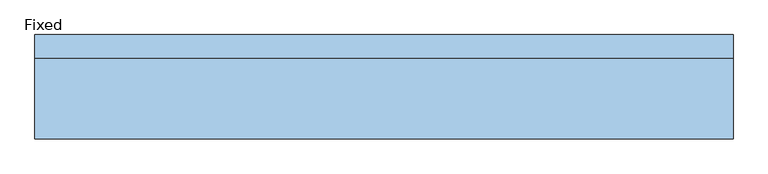
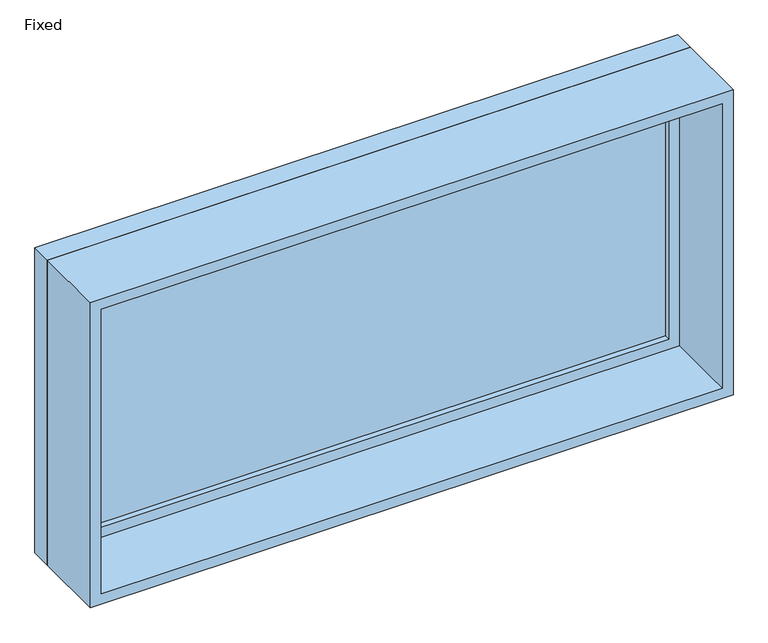
"""IFC4 building model written with IfcOpenShell, lengths in millimetres: window geometry, Fixed."""

import ifcopenshell
import ifcopenshell.guid

model = None  # the IFC model being written
_history = None  # IfcOwnerHistory: only IFC2X3 demands one
_inside = {}  # id of a spatial element -> (the spatial element, [elements in it])
_under = {}  # id of a project, library or spatial element -> (it, [spatial elements below it])
_declared = {}  # id of a project -> (the project, [libraries it declares])
_typed = {}  # id of a type object -> (the type object, [elements of that type])
_made_of = {}  # id of a material, layer set ... -> (it, [elements and type objects made of it])


def new_model(schema):
    """Start an empty IFC model of exactly this schema.

    Asked for "IFC4X3", IfcOpenShell would pick the latest addendum, in which some entities
    have other attributes; the version numbers below select the first issue.
    IFC2X3 requires an IfcOwnerHistory on every rooted entity: one is made here for all.
    """
    global model, _history
    if schema == "IFC4X3":
        model = ifcopenshell.file(schema_version=(4, 3, 0, 0))
    else:
        model = ifcopenshell.file(schema=schema)
    _inside.clear()
    _under.clear()
    _declared.clear()
    _typed.clear()
    _made_of.clear()
    _history = None
    if model.schema == "IFC2X3":
        org = make("IfcOrganization", Name="unknown")
        user = make(
            "IfcPersonAndOrganization",
            ThePerson=make("IfcPerson", FamilyName="unknown"),
            TheOrganization=org,
        )
        app = make(
            "IfcApplication",
            ApplicationDeveloper=org,
            Version="unknown",
            ApplicationFullName="unknown",
            ApplicationIdentifier="unknown",
        )
        _history = make(
            "IfcOwnerHistory",
            OwningUser=user,
            OwningApplication=app,
            ChangeAction="ADDED",
            CreationDate=0,
        )
    return model


def make(cls, **values):
    """One entity of the class cls with the attributes given. An attribute that is None is left unset."""
    return model.create_entity(
        cls, **{name: value for name, value in values.items() if value is not None}
    )


def rooted(cls, **values):
    """An entity with a GlobalId (a new one), such as an element, a storey or a relation."""
    return make(cls, GlobalId=ifcopenshell.guid.new(), OwnerHistory=_history, **values)


def si_unit(unit_type, name, prefix=None):
    """IfcSIUnit, for example si_unit("LENGTHUNIT", "METRE", prefix="MILLI")."""
    return make("IfcSIUnit", UnitType=unit_type, Prefix=prefix, Name=name)


def assignment(units):
    """IfcUnitAssignment: the units of a project."""
    return None if units is None else make("IfcUnitAssignment", Units=units)


def point(xyz):
    """IfcCartesianPoint."""
    return None if xyz is None else make("IfcCartesianPoint", Coordinates=xyz)


def direction(xyz):
    """IfcDirection."""
    return None if xyz is None else make("IfcDirection", DirectionRatios=xyz)


def frame(location, z_axis=None, x_axis=None):
    """IfcAxis2Placement3D, a coordinate frame: its origin and axes. An axis left out is left unset."""
    return make(
        "IfcAxis2Placement3D",
        Location=point(location),
        Axis=direction(z_axis),
        RefDirection=direction(x_axis),
    )


def origin():
    """The frame at (0, 0, 0) with its axes left unset."""
    return frame((0.0, 0.0, 0.0))


def place(relative_to, where):
    """IfcLocalPlacement: puts the frame where relative to a parent placement (None: the world)."""
    return make(
        "IfcLocalPlacement", PlacementRelTo=relative_to, RelativePlacement=where
    )


def context(
    kind, dimensions, precision=None, world=None, true_north=None, identifier=None
):
    """IfcGeometricRepresentationContext, for example the 3D "Model" context."""
    return make(
        "IfcGeometricRepresentationContext",
        ContextIdentifier=identifier,
        ContextType=kind,
        CoordinateSpaceDimension=dimensions,
        Precision=precision,
        WorldCoordinateSystem=world,
        TrueNorth=true_north,
    )


def project(units=None, contexts=None):
    """IfcProject with its units and contexts."""
    return rooted(
        "IfcProject",
        Name="project",
        RepresentationContexts=contexts,
        UnitsInContext=assignment(units),
    )


def spatial(cls, under=None, at=None, **own):
    """A site, building, storey or space (cls), placed at a placement, below another one or the project."""
    s = rooted(cls, ObjectPlacement=at, **own)
    if under is not None:
        _under.setdefault(under.id(), (under, []))[1].append(s)
    return s


def polyline(points):
    """IfcPolyline through the points."""
    return make("IfcPolyline", Points=[point(p) for p in points])


def outline(outer, holes=None, kind="AREA"):
    """IfcArbitraryClosedProfileDef: a profile drawn as a closed curve; with holes, ...WithVoids."""
    if holes is None:
        return make("IfcArbitraryClosedProfileDef", ProfileType=kind, OuterCurve=outer)
    return make(
        "IfcArbitraryProfileDefWithVoids",
        ProfileType=kind,
        OuterCurve=outer,
        InnerCurves=holes,
    )


def extrude(swept, where, along, depth):
    """IfcExtrudedAreaSolid: the profile swept, set in the frame where, extruded along a direction by depth."""
    return make(
        "IfcExtrudedAreaSolid",
        SweptArea=swept,
        Position=where,
        ExtrudedDirection=direction(along),
        Depth=depth,
    )


def shape(context_of_items, identifier, shape_type, items):
    """IfcShapeRepresentation: the items that make up one representation, for example the "Body"."""
    return make(
        "IfcShapeRepresentation",
        ContextOfItems=context_of_items,
        RepresentationIdentifier=identifier,
        RepresentationType=shape_type,
        Items=items,
    )


def source(mapping_origin, context_of_items, identifier, shape_type, items):
    """IfcRepresentationMap: a shape defined once, which mapped items show again and again."""
    return make(
        "IfcRepresentationMap",
        MappingOrigin=mapping_origin,
        MappedRepresentation=shape(context_of_items, identifier, shape_type, items),
    )


def transform(
    local_origin,
    x_axis=None,
    y_axis=None,
    z_axis=None,
    scale=None,
    scale2=None,
    scale3=None,
    uniform=True,
):
    """IfcCartesianTransformationOperator3D, or its non-uniform kind. x_axis, y_axis, z_axis: its Axis1, 2, 3."""
    if uniform:
        return make(
            "IfcCartesianTransformationOperator3D",
            Axis1=direction(x_axis),
            Axis2=direction(y_axis),
            LocalOrigin=point(local_origin),
            Scale=scale,
            Axis3=direction(z_axis),
        )
    return make(
        "IfcCartesianTransformationOperator3DnonUniform",
        Axis1=direction(x_axis),
        Axis2=direction(y_axis),
        LocalOrigin=point(local_origin),
        Scale=scale,
        Axis3=direction(z_axis),
        Scale2=scale2,
        Scale3=scale3,
    )


def mapped(mapping_source, mapping_target):
    """IfcMappedItem: shows the shape of a source again, moved by a transform."""
    return make(
        "IfcMappedItem", MappingSource=mapping_source, MappingTarget=mapping_target
    )


def made_of(thing, what):
    """Note that an element or type object is made of a material, layer set ...; save() writes the relation."""
    if what is not None:
        _made_of.setdefault(what.id(), (what, []))[1].append(thing)
    return thing


def element(
    cls,
    number,
    at=None,
    inside=None,
    cuts=None,
    type_object=None,
    material=None,
    context=None,
    identifier="Body",
    shape_type=None,
    held_by="IfcProductDefinitionShape",
    body=None,
    shapes=None,
    **own,
):
    """One element of the class cls, such as IfcWall. Its Tag is "e" and its number.

    at: its placement. inside: the storey or other place that contains it. cuts: it is an
    opening in that element (IfcRelVoidsElement). A single representation is given by context,
    identifier, shape_type and body (its items); several are given by shapes. held_by: the class
    of the entity that holds the representations. save() writes the other relations.
    """
    e = rooted(cls, Tag="e%d" % number, ObjectPlacement=at, **own)
    if body is not None:
        shapes = [shape(context, identifier, shape_type, body)]
    if shapes is not None:
        e.Representation = make(held_by, Representations=shapes)
    if inside is not None:
        _inside.setdefault(inside.id(), (inside, []))[1].append(e)
    if cuts is not None:
        rooted(
            "IfcRelVoidsElement", RelatingBuildingElement=cuts, RelatedOpeningElement=e
        )
    if type_object is not None:
        _typed.setdefault(type_object.id(), (type_object, []))[1].append(e)
    return made_of(e, material)


def aggregate(whole, parts):
    """IfcRelAggregates: a whole, such as a stair, and the parts it consists of."""
    return rooted("IfcRelAggregates", RelatingObject=whole, RelatedObjects=parts)


def save(model, path):
    """Write the relations noted so far, then the file.

    IfcRelAggregates (storeys below a building ...), IfcRelContainedInSpatialStructure (elements
    in a storey), IfcRelDefinesByType, IfcRelAssociatesMaterial and IfcRelDeclares: one each for
    every whole, place, type object, material and project.
    """
    for whole, parts in _under.values():
        aggregate(whole, parts)
    for where, things in _inside.values():
        rooted(
            "IfcRelContainedInSpatialStructure",
            RelatedElements=things,
            RelatingStructure=where,
        )
    for kind, things in _typed.values():
        rooted("IfcRelDefinesByType", RelatedObjects=things, RelatingType=kind)
    for what, things in _made_of.values():
        rooted("IfcRelAssociatesMaterial", RelatedObjects=things, RelatingMaterial=what)
    for by, libraries in _declared.values():
        rooted("IfcRelDeclares", RelatingContext=by, RelatedDefinitions=libraries)
    model.write(path)


def fixed_b37ba2c0(model_context):
    return source(origin(), model_context, "Body", "SweptSolid", [
        extrude(outline(polyline([(835.025, 92.075), (-911.225, 92.075), (-911.225, 104.775), (835.025, 104.775), (835.025, 92.075)])), frame((0.0, 0.0, 1257.3), z_axis=(0.0, 0.0, 1.0), x_axis=(1.0, 0.0, 0.0)), (0.0, 0.0, 1.0), 812.8),
        extrude(outline(polyline([(2114.55, -955.675), (1212.85, -955.675), (1212.85, 879.475), (2114.55, 879.475), (2114.55, -955.675)]), holes=[polyline([(2070.1, -911.225), (2070.1, 835.025), (1257.3, 835.025), (1257.3, -911.225), (2070.1, -911.225)])]), frame((0.0, 76.2, 0.0), z_axis=(0.0, 1.0, 0.0), x_axis=(0.0, 0.0, 1.0)), (0.0, 0.0, 1.0), 44.45),
        extrude(outline(polyline([(2133.6, -974.725), (1193.8, -974.725), (1193.8, 898.525), (2133.6, 898.525), (2133.6, -974.725)]), holes=[polyline([(2101.85, -942.975), (2101.85, 866.775), (1225.55, 866.775), (1225.55, -942.975), (2101.85, -942.975)])]), frame((0.0, -139.7, 0.0), z_axis=(0.0, 1.0, 0.0), x_axis=(0.0, 0.0, 1.0)), (0.0, 0.0, 1.0), 215.9),
        extrude(outline(polyline([(2133.6, 898.525), (2133.6, -974.725), (1193.8, -974.725), (1193.8, 898.525), (2133.6, 898.525)]), holes=[polyline([(2114.55, 879.475), (1212.85, 879.475), (1212.85, -955.675), (2114.55, -955.675), (2114.55, 879.475)])]), frame((0.0, 76.2, 0.0), z_axis=(0.0, 1.0, 0.0), x_axis=(0.0, 0.0, 1.0)), (0.0, 0.0, 1.0), 63.5),
    ])


if __name__ == "__main__":
    model = new_model("IFC4")
    model_context = context("Model", 3, world=origin())
    ifc_project = project(units=[si_unit("LENGTHUNIT", "METRE", prefix="MILLI")], contexts=[model_context])
    site = spatial("IfcSite", under=ifc_project)
    building = spatial("IfcBuilding", under=site)
    placement = place(None, origin())
    fixed_shape = fixed_b37ba2c0(model_context)
    element("IfcWindow", 1, ObjectType="Fixed : 6' 1 34\"\" x 3' 1\"", at=placement, inside=building, context=model_context, shape_type="MappedRepresentation", body=[
        mapped(fixed_shape, transform((0.0, 0.0, 0.0), x_axis=(1.0, 0.0, 0.0), y_axis=(0.0, 1.0, 0.0), z_axis=(0.0, 0.0, 1.0))),
    ])
    save(model, "model.ifc")

# Revit data of these elements
# Type "Fixed : 6' 1 34\"\" x 3' 1\""
#   Type Mark = "10"
#   Assembly Code = "B2020100"
#   Height = 3' - 1"
#   Default Sill Height = 3' - 11"
#   Width = 6' - 1 3/4"
#   Window Inset = 0' - 0 3/4"
#   Glass Pane Material = Glass
#   Sash Material = accent 2
#   Wall Closure = (empty or 0)
# Element 1 (IfcWindow, "Fixed : 6' 1 34\"\" x 3' 1\"")
#   Materials on its faces: "accent 2", "Glass"
# Materials
#   "Glass": class "Glass", colour RGB 236 240 239, transparency 0.85, Description = "Soda Lime Glass", Cost = 0
#   "accent 2": class "Wood", colour RGB 80 80 80, transparency 0, Description = "Wood framing, thermal airspace", Cost = 0
